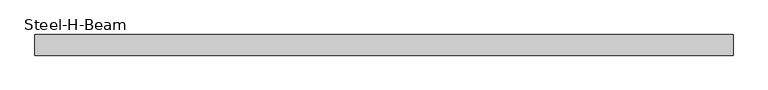
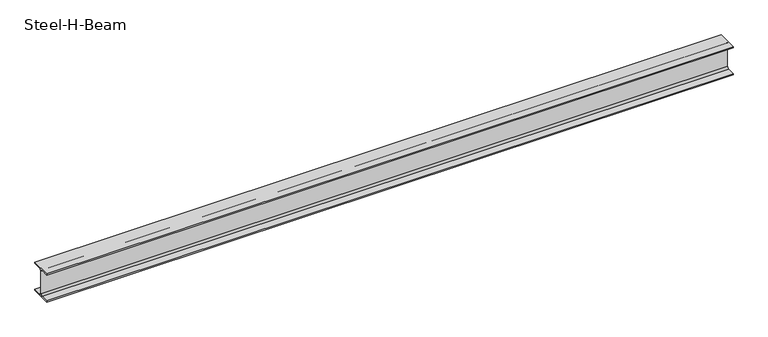
"""IFC4 building model written with IfcOpenShell, lengths in millimetres: beam geometry, Steel-H-Beam : BM121_H-294×200x8x12."""

from ifc_helpers import new_model, si_unit, point, frame, frame_2d, origin, place, context, project, spatial, polyline, circle_curve, trimmed, segment, composite_curve, outline, extrude, source, transform, mapped, element, save


def steel_h_beam_4d9bb108(model_context):
    return source(origin(), model_context, "Body", "SweptSolid", [
        extrude(outline(composite_curve([segment(polyline([(100.0, -135.0), (100.0, -147.0), (-100.0, -147.0), (-100.0, -135.0), (-22.0, -135.0)]), True, "CONTINUOUS"), segment(trimmed(circle_curve(frame_2d((-22.0, -117.0)), 18.0), [point((-22.0, -135.0))], [point((-4.0, -117.0))], True, "CARTESIAN"), True, "CONTINUOUS"), segment(polyline([(-4.0, -117.0), (-4.0, 117.0)]), True, "CONTINUOUS"), segment(trimmed(circle_curve(frame_2d((-22.0, 117.0)), 18.0), [point((-4.0, 117.0))], [point((-22.0, 135.0))], True, "CARTESIAN"), True, "CONTINUOUS"), segment(polyline([(-22.0, 135.0), (-100.0, 135.0), (-100.0, 147.0), (100.0, 147.0), (100.0, 135.0), (22.0, 135.0)]), True, "CONTINUOUS"), segment(trimmed(circle_curve(frame_2d((22.0, 117.0)), 18.0), [point((22.0, 135.0))], [point((4.0, 117.0))], True, "CARTESIAN"), True, "CONTINUOUS"), segment(polyline([(4.0, 117.0), (4.0, -117.0)]), True, "CONTINUOUS"), segment(trimmed(circle_curve(frame_2d((22.0, -117.0)), 18.0), [point((4.0, -117.0))], [point((22.0, -135.0))], True, "CARTESIAN"), True, "CONTINUOUS"), segment(polyline([(22.0, -135.0), (100.0, -135.0)]), True, "CONTINUOUS")], self_intersect=False)), frame((-3390.0, 0.0, 0.0), z_axis=(1.0, 0.0, 0.0), x_axis=(0.0, 1.0, 0.0)), (0.0, 0.0, 1.0), 6780.0),
    ])


if __name__ == "__main__":
    model = new_model("IFC4")
    model_context = context("Model", 3, world=origin())
    ifc_project = project(units=[si_unit("LENGTHUNIT", "METRE", prefix="MILLI")], contexts=[model_context])
    site = spatial("IfcSite", under=ifc_project)
    building = spatial("IfcBuilding", under=site)
    placement = place(None, origin())
    steel_h_beam_shape = steel_h_beam_4d9bb108(model_context)
    element("IfcBeam", 1, ObjectType="Steel-H-Beam : BM121_H-294×200x8x12", at=placement, inside=building, context=model_context, shape_type="MappedRepresentation", body=[
        mapped(steel_h_beam_shape, transform((0.0, 0.0, 0.0), x_axis=(1.0, 0.0, 0.0), y_axis=(0.0, 1.0, 0.0), z_axis=(0.0, 0.0, 1.0))),
    ])
    save(model, "model.ifc")

# Revit data of these elements
# Type "Steel-H-Beam : BM121_H-294×200x8x12"
#   Surface Area = 1.3411 m²/m
#   Section Area = 72.3812 cm²
#   Mass per Unit Length = 56.8193 kg/m
#   Length [instance default] = 3000 mm
#   B = 200 mm
#   H = 294 mm
#   r = 18 mm
#   tw = 8 mm
#   tf = 12 mm
#   hec_material4 [instance default] = none
#   hec_material3 [instance default] = none
#   hec_material2 [instance default] = none
#   hec_material1 [instance default] = none
#   Structural Material [instance default] = Steel, 45-345
#   Assembly Code = ""
# Element 1 (IfcBeam, "Steel-H-Beam : BM121_H-294×200x8x12")
#   hec_material3 = F01AC000-00002_Building/Shelter Fire Proofing Work_Intumescent Coating Type_1 hr. rating (UL 1709))
#   hec_material2 = S01AA010-00002_Main Steel Structure Fabrication Work_Shelter/Building_Steel Painting/Coating_for Fireproofed Steel Surface, Surface Preparation & Primer Coat
#   hec_material1 = S03AA028-00001_Main Steel Structure Erection Work_Shelter/Building_Medium Steel
#   Structural Material = S01AA002-00001_Main Steel Structure Fabrication Work_Shelter/Building_Medium Steel - Standard
#   Materials on its faces: "S01AA002-00001_Main Steel Structure Fabrication Work_Shelter/Building_Medium Steel - Standard"
# Materials
#   "Steel, 45-345": class "Metal", colour RGB 189 187 185, transparency 0, Description = "Steel 345 MPa", Cost = 0
#   "S01AA002-00001_Main Steel Structure Fabrication Work_Shelter/Building_Medium Steel - Standard": class "Metal", colour RGB 120 120 120, transparency 0, Comments = "(90KG/M>Weight≥30KG/M)", Description = "Structural steel 50ksi", W00) Work Master Code = "S01AA002-0001", W01) Work Master_Lv1 = "Main Steel Structure Fabrication Work", W02) Work Master_Lv2 = "Shelter/Building", W03) Work Master_Spec.1 = "Medium Steel - Standard (90KG/M>Weight≥30KG/M)", Cost = 0
#   "F01AC000-00002_Building/Shelter Fire Proofing Work_Intumescent Coating Type_1 hr. rating (UL 1709))": class "Metal", colour RGB 255 128 128, transparency 0, Description = "Paint finished steel", W00) Work Master Code = "F01AC000-00002", W01) Work Master_Lv1 = "Building/Shelter Fire Proofing Work", W02) Work Master_Lv2 = "Intumescent Coating Type", W03) Work Master_Spec.1 = "1 hr. rating (UL 1709)", Cost = 0
#   "S01AA010-00002_Main Steel Structure Fabrication Work_Shelter/Building_Steel Painting/Coating_for Fireproofed Steel Surface, Surface Preparation & Primer Coat": class "Metal", colour RGB 120 120 120, transparency 0, Description = "Paint finished steel", W00) Work Master Code = "SS01AA010-00002", W01) Work Master_Lv1 = "Main Steel Structure Fabrication Work", W02) Work Master_Lv2 = "Shelter/Building", W03) Work Master_Spec.1 = "Steel Painting/Coating", W04) Work Master_Spec.2 = "for Fireproofed Steel Surface, Surface Preparation & Primer Coat", Cost = 0
#   "S03AA028-00001_Main Steel Structure Erection Work_Shelter/Building_Medium Steel": class "Metal", colour RGB 120 120 120, transparency 0, Comments = "(90KG/M>Weight≥30KG/M)", Description = "Structural steel 50ksi", W00) Work Master Code = "S03AA028-0001", W01) Work Master_Lv1 = "Main Steel Structure Erection Work", W02) Work Master_Lv2 = "Shelter/Building", W03) Work Master_Spec.1 = "Medium Steel (90KG/M>Weight≥30KG/M)", Cost = 0
